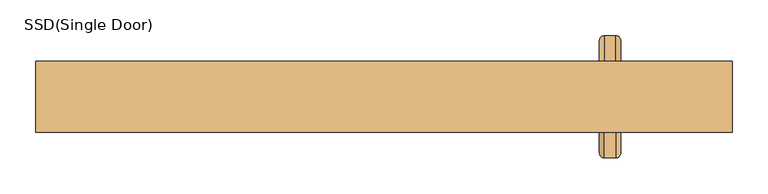
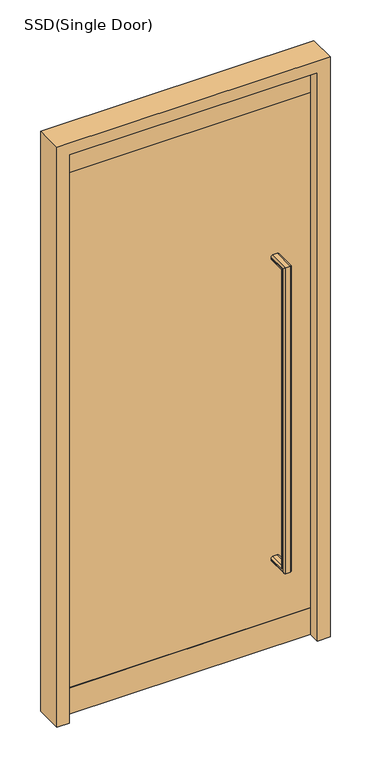
"""IFC4 building model written with IfcOpenShell, lengths in millimetres: door geometry, SSD(Single Door) : H_DR_AR B12_Door_Single_Glass_W1000xH2200_SSD-1."""

from ifc_helpers import new_model, si_unit, frame, origin, origin_with_axes, place, context, project, spatial, polyline, circle_curve, ellipse_curve, outline, extrude, source, transform, mapped, element, save
from ifc_brep_helpers import plane_surface, cylinder_surface, advanced_brep


def ssd_single_door_d0e6de12(model_context):
    return source(origin(), model_context, "Body", "SolidModel", [
        extrude(outline(polyline([(0.0, -490.0), (0.0, -445.0), (2155.0, -445.0), (2155.0, 445.0), (0.0, 445.0), (0.0, 490.0), (2200.0, 490.0), (2200.0, -490.0), (0.0, -490.0)])), frame((0.0, 5.0, 0.0), z_axis=(0.0, 1.0, 0.0), x_axis=(0.0, 0.0, 1.0)), (0.0, 0.0, 1.0), 100.0),
        advanced_brep(
        [(310.0, 49.0, 1485.0), (326.0, 49.0, 1485.0), (333.0, 49.0, 1478.0), (333.0, 49.0, 1475.0), (326.0, 49.0, 1468.0), (310.0, 49.0, 1468.0), (303.0, 49.0, 1475.0), (303.0, 49.0, 1478.0), (310.0, 49.0, 325.0), (303.0, 49.0, 332.0), (303.0, 49.0, 335.0), (310.0, 49.0, 342.0), (326.0, 49.0, 342.0), (333.0, 49.0, 335.0), (333.0, 49.0, 332.0), (326.0, 49.0, 325.0), (310.0, -31.0, 1485.0), (326.0, -31.0, 1485.0), (333.0, -24.0, 1478.0), (333.0, -24.0, 332.0), (333.0, -21.0, 335.0), (333.0, -21.0, 1475.0), (326.0, -14.0, 1468.0), (310.0, -14.0, 1468.0), (303.0, -21.0, 1475.0), (303.0, -21.0, 335.0), (303.0, -24.0, 332.0), (303.0, -24.0, 1478.0), (310.0, -31.0, 325.0), (326.0, -31.0, 325.0), (326.0, -14.0, 342.0), (310.0, -14.0, 342.0)],
        [
            (0, 1),
            (1, 2, circle_curve(frame((326.0, 49.0, 1478.0), z_axis=(0.0, 1.0, 0.0), x_axis=(0.0, 0.0, -1.0)), 7.0)),
            (2, 3),
            (3, 4, circle_curve(frame((326.0, 49.0, 1475.0), z_axis=(0.0, 1.0, 0.0), x_axis=(0.0, 0.0, -1.0)), 7.0)),
            (4, 5),
            (5, 6, circle_curve(frame((310.0, 49.0, 1475.0), z_axis=(0.0, 1.0, 0.0), x_axis=(0.0, 0.0, -1.0)), 7.0)),
            (6, 7),
            (7, 0, circle_curve(frame((310.0, 49.0, 1478.0), z_axis=(0.0, 1.0, 0.0), x_axis=(0.0, 0.0, -1.0)), 7.0)),
            (8, 9, circle_curve(frame((310.0, 49.0, 332.0), z_axis=(0.0, 1.0, 0.0), x_axis=(0.0, 0.0, 1.0)), 7.0)),
            (9, 10),
            (10, 11, circle_curve(frame((310.0, 49.0, 335.0), z_axis=(0.0, 1.0, 0.0), x_axis=(0.0, 0.0, 1.0)), 7.0)),
            (11, 12),
            (12, 13, circle_curve(frame((326.0, 49.0, 335.0), z_axis=(0.0, 1.0, 0.0), x_axis=(0.0, 0.0, 1.0)), 7.0)),
            (13, 14),
            (14, 15, circle_curve(frame((326.0, 49.0, 332.0), z_axis=(0.0, 1.0, 0.0), x_axis=(0.0, 0.0, 1.0)), 7.0)),
            (15, 8),
            (0, 16),
            (16, 17),
            (17, 1),
            (17, 18, ellipse_curve(frame((326.0, -24.0, 1478.0), z_axis=(0.0, 0.7071067811865475, 0.7071067811865475), x_axis=(0.0, 0.7071067811865476, -0.7071067811865474)), 9.8994949, 7.0)),
            (18, 2),
            (18, 19),
            (19, 14),
            (13, 20),
            (20, 21),
            (21, 3),
            (21, 22, ellipse_curve(frame((326.0, -21.0, 1475.0), z_axis=(0.0, 0.7071067811865475, 0.7071067811865475), x_axis=(0.0, 0.7071067811865476, -0.7071067811865474)), 9.8994949, 7.0)),
            (22, 4),
            (22, 23),
            (23, 5),
            (23, 24, ellipse_curve(frame((310.0, -21.0, 1475.0), z_axis=(0.0, 0.7071067811865475, 0.7071067811865475), x_axis=(0.0, 0.7071067811865476, -0.7071067811865474)), 9.8994949, 7.0)),
            (24, 6),
            (24, 25),
            (25, 10),
            (9, 26),
            (26, 27),
            (27, 7),
            (27, 16, ellipse_curve(frame((310.0, -24.0, 1478.0), z_axis=(0.0, 0.7071067811865475, 0.7071067811865475), x_axis=(0.0, 0.7071067811865476, -0.7071067811865474)), 9.8994949, 7.0)),
            (16, 28),
            (28, 29),
            (29, 17),
            (29, 19, ellipse_curve(frame((326.0, -24.0, 332.0), z_axis=(0.0, -0.7071067811865475, 0.7071067811865475), x_axis=(0.0, 0.7071067811865474, 0.7071067811865476)), 9.8994949, 7.0)),
            (20, 30, ellipse_curve(frame((326.0, -21.0, 335.0), z_axis=(0.0, -0.7071067811865475, 0.7071067811865475), x_axis=(0.0, 0.7071067811865474, 0.7071067811865476)), 9.8994949, 7.0)),
            (30, 22),
            (30, 31),
            (31, 23),
            (31, 25, ellipse_curve(frame((310.0, -21.0, 335.0), z_axis=(0.0, -0.7071067811865475, 0.7071067811865475), x_axis=(0.0, 0.7071067811865474, 0.7071067811865476)), 9.8994949, 7.0)),
            (26, 28, ellipse_curve(frame((310.0, -24.0, 332.0), z_axis=(0.0, -0.7071067811865475, 0.7071067811865475), x_axis=(0.0, 0.7071067811865474, 0.7071067811865476)), 9.8994949, 7.0)),
            (28, 8),
            (15, 29),
            (12, 30),
            (11, 31),
        ],
        [
            plane_surface(frame((0.0, 49.0, 1485.0), z_axis=(0.0, 1.0, 0.0), x_axis=(1.0, 0.0, 0.0))),
            plane_surface(frame((0.0, 49.0, 325.0), z_axis=(0.0, 1.0, 0.0), x_axis=(1.0, 0.0, 0.0))),
            plane_surface(frame((310.0, 49.0, 1485.0), z_axis=(0.0, 0.0, 1.0), x_axis=(0.0, -1.0, 0.0))),
            cylinder_surface(frame((326.0, 49.0, 1478.0), z_axis=(0.0, 1.0, 0.0), x_axis=(0.0, 0.0, -1.0)), 7.0),
            plane_surface(frame((333.0, 49.0, 1478.0), z_axis=(1.0, 0.0, 0.0), x_axis=(0.0, -1.0, 0.0))),
            cylinder_surface(frame((326.0, 49.0, 1475.0), z_axis=(0.0, 1.0, 0.0), x_axis=(0.0, 0.0, -1.0)), 7.0),
            plane_surface(frame((326.0, 49.0, 1468.0), z_axis=(0.0, 0.0, -1.0), x_axis=(0.0, -1.0, 0.0))),
            cylinder_surface(frame((310.0, 49.0, 1475.0), z_axis=(0.0, 1.0, 0.0), x_axis=(0.0, 0.0, -1.0)), 7.0),
            plane_surface(frame((303.0, 49.0, 1475.0), z_axis=(-1.0, 0.0, 0.0), x_axis=(0.0, -1.0, 0.0))),
            cylinder_surface(frame((310.0, 49.0, 1478.0), z_axis=(0.0, 1.0, 0.0), x_axis=(0.0, 0.0, -1.0)), 7.0),
            plane_surface(frame((310.0, -31.0, 1485.0), z_axis=(0.0, -1.0, 0.0), x_axis=(0.0, 0.0, -1.0))),
            cylinder_surface(frame((326.0, -24.0, 1485.0), z_axis=(0.0, 0.0, 1.0), x_axis=(0.0, 1.0, 0.0)), 7.0),
            cylinder_surface(frame((326.0, -21.0, 1485.0), z_axis=(0.0, 0.0, 1.0), x_axis=(0.0, 1.0, 0.0)), 7.0),
            plane_surface(frame((326.0, -14.0, 1468.0), z_axis=(0.0, 1.0, 0.0), x_axis=(0.0, 0.0, -1.0))),
            cylinder_surface(frame((310.0, -21.0, 1485.0), z_axis=(0.0, 0.0, 1.0), x_axis=(0.0, 1.0, 0.0)), 7.0),
            cylinder_surface(frame((310.0, -24.0, 1485.0), z_axis=(0.0, 0.0, 1.0), x_axis=(0.0, 1.0, 0.0)), 7.0),
            plane_surface(frame((310.0, -31.0, 325.0), z_axis=(0.0, 0.0, -1.0), x_axis=(0.0, 1.0, 0.0))),
            cylinder_surface(frame((326.0, -31.0, 332.0), z_axis=(0.0, -1.0, 0.0), x_axis=(0.0, 0.0, 1.0)), 7.0),
            cylinder_surface(frame((326.0, -31.0, 335.0), z_axis=(0.0, -1.0, 0.0), x_axis=(0.0, 0.0, 1.0)), 7.0),
            plane_surface(frame((326.0, -14.0, 342.0), z_axis=(0.0, 0.0, 1.0), x_axis=(0.0, 1.0, 0.0))),
            cylinder_surface(frame((310.0, -31.0, 335.0), z_axis=(0.0, -1.0, 0.0), x_axis=(0.0, 0.0, 1.0)), 7.0),
            cylinder_surface(frame((310.0, -31.0, 332.0), z_axis=(0.0, -1.0, 0.0), x_axis=(0.0, 0.0, 1.0)), 7.0),
        ],
        [
            (0, [[1, 2, 3, 4, 5, 6, 7, 8]]),
            (1, [[9, 10, 11, 12, 13, 14, 15, 16]]),
            (2, [[-1, 17, 18, 19]]),
            (3, [[-2, -19, 20, 21]]),
            (4, [[-3, -21, 22, 23, -14, 24, 25, 26]]),
            (5, [[-4, -26, 27, 28]]),
            (6, [[-5, -28, 29, 30]]),
            (7, [[-6, -30, 31, 32]]),
            (8, [[-7, -32, 33, 34, -10, 35, 36, 37]]),
            (9, [[-8, -37, 38, -17]]),
            (10, [[-18, 39, 40, 41]]),
            (11, [[-20, -41, 42, -22]]),
            (12, [[-27, -25, 43, 44]]),
            (13, [[-29, -44, 45, 46]]),
            (14, [[-31, -46, 47, -33]]),
            (15, [[-38, -36, 48, -39]]),
            (16, [[-40, 49, -16, 50]]),
            (17, [[-42, -50, -15, -23]]),
            (18, [[-43, -24, -13, 51]]),
            (19, [[-45, -51, -12, 52]]),
            (20, [[-47, -52, -11, -34]]),
            (21, [[-48, -35, -9, -49]]),
        ],
    ),
        advanced_brep(
        [(310.0, 61.0, 1485.0), (303.0, 61.0, 1478.0), (303.0, 61.0, 1475.0), (310.0, 61.0, 1468.0), (326.0, 61.0, 1468.0), (333.0, 61.0, 1475.0), (333.0, 61.0, 1478.0), (326.0, 61.0, 1485.0), (310.0, 61.0, 325.0), (326.0, 61.0, 325.0), (333.0, 61.0, 332.0), (333.0, 61.0, 335.0), (326.0, 61.0, 342.0), (310.0, 61.0, 342.0), (303.0, 61.0, 335.0), (303.0, 61.0, 332.0), (310.0, 141.0, 1485.0), (303.0, 134.0, 1478.0), (303.0, 134.0, 332.0), (303.0, 131.0, 335.0), (303.0, 131.0, 1475.0), (310.0, 124.0, 1468.0), (326.0, 124.0, 1468.0), (333.0, 131.0, 1475.0), (333.0, 131.0, 335.0), (333.0, 134.0, 332.0), (333.0, 134.0, 1478.0), (326.0, 141.0, 1485.0), (310.0, 141.0, 325.0), (310.0, 124.0, 342.0), (326.0, 124.0, 342.0), (326.0, 141.0, 325.0)],
        [
            (0, 1, circle_curve(frame((310.0, 61.0, 1478.0), z_axis=(0.0, -1.0, 0.0), x_axis=(0.0, 0.0, 1.0)), 7.0)),
            (1, 2),
            (2, 3, circle_curve(frame((310.0, 61.0, 1475.0), z_axis=(0.0, -1.0, 0.0), x_axis=(0.0, 0.0, 1.0)), 7.0)),
            (3, 4),
            (4, 5, circle_curve(frame((326.0, 61.0, 1475.0), z_axis=(0.0, -1.0, 0.0), x_axis=(0.0, 0.0, 1.0)), 7.0)),
            (5, 6),
            (6, 7, circle_curve(frame((326.0, 61.0, 1478.0), z_axis=(0.0, -1.0, 0.0), x_axis=(0.0, 0.0, 1.0)), 7.0)),
            (7, 0),
            (8, 9),
            (9, 10, circle_curve(frame((326.0, 61.0, 332.0), z_axis=(0.0, -1.0, 0.0), x_axis=(0.0, 0.0, -1.0)), 7.0)),
            (10, 11),
            (11, 12, circle_curve(frame((326.0, 61.0, 335.0), z_axis=(0.0, -1.0, 0.0), x_axis=(0.0, 0.0, -1.0)), 7.0)),
            (12, 13),
            (13, 14, circle_curve(frame((310.0, 61.0, 335.0), z_axis=(0.0, -1.0, 0.0), x_axis=(0.0, 0.0, -1.0)), 7.0)),
            (14, 15),
            (15, 8, circle_curve(frame((310.0, 61.0, 332.0), z_axis=(0.0, -1.0, 0.0), x_axis=(0.0, 0.0, -1.0)), 7.0)),
            (0, 16),
            (16, 17, ellipse_curve(frame((310.0, 134.0, 1478.0), z_axis=(0.0, -0.7071067811865475, 0.7071067811865475), x_axis=(0.0, -0.7071067811865476, -0.7071067811865474)), 9.8994949, 7.0)),
            (17, 1),
            (17, 18),
            (18, 15),
            (14, 19),
            (19, 20),
            (20, 2),
            (20, 21, ellipse_curve(frame((310.0, 131.0, 1475.0), z_axis=(0.0, -0.7071067811865475, 0.7071067811865475), x_axis=(0.0, -0.7071067811865476, -0.7071067811865474)), 9.8994949, 7.0)),
            (21, 3),
            (21, 22),
            (22, 4),
            (22, 23, ellipse_curve(frame((326.0, 131.0, 1475.0), z_axis=(0.0, -0.7071067811865475, 0.7071067811865475), x_axis=(0.0, -0.7071067811865476, -0.7071067811865474)), 9.8994949, 7.0)),
            (23, 5),
            (23, 24),
            (24, 11),
            (10, 25),
            (25, 26),
            (26, 6),
            (26, 27, ellipse_curve(frame((326.0, 134.0, 1478.0), z_axis=(0.0, -0.7071067811865475, 0.7071067811865475), x_axis=(0.0, -0.7071067811865476, -0.7071067811865474)), 9.8994949, 7.0)),
            (27, 7),
            (27, 16),
            (16, 28),
            (28, 18, ellipse_curve(frame((310.0, 134.0, 332.0), z_axis=(0.0, 0.7071067811865475, 0.7071067811865475), x_axis=(0.0, -0.7071067811865474, 0.7071067811865476)), 9.8994949, 7.0)),
            (19, 29, ellipse_curve(frame((310.0, 131.0, 335.0), z_axis=(0.0, 0.7071067811865475, 0.7071067811865475), x_axis=(0.0, -0.7071067811865474, 0.7071067811865476)), 9.8994949, 7.0)),
            (29, 21),
            (29, 30),
            (30, 22),
            (30, 24, ellipse_curve(frame((326.0, 131.0, 335.0), z_axis=(0.0, 0.7071067811865475, 0.7071067811865475), x_axis=(0.0, -0.7071067811865474, 0.7071067811865476)), 9.8994949, 7.0)),
            (25, 31, ellipse_curve(frame((326.0, 134.0, 332.0), z_axis=(0.0, 0.7071067811865475, 0.7071067811865475), x_axis=(0.0, -0.7071067811865474, 0.7071067811865476)), 9.8994949, 7.0)),
            (31, 27),
            (31, 28),
            (28, 8),
            (13, 29),
            (12, 30),
            (9, 31),
        ],
        [
            plane_surface(frame((0.0, 61.0, 1485.0), z_axis=(0.0, -1.0, 0.0), x_axis=(1.0, 0.0, 0.0))),
            plane_surface(frame((0.0, 61.0, 325.0), z_axis=(0.0, -1.0, 0.0), x_axis=(1.0, 0.0, 0.0))),
            cylinder_surface(frame((310.0, 61.0, 1478.0), z_axis=(0.0, -1.0, 0.0), x_axis=(0.0, 0.0, 1.0)), 7.0),
            plane_surface(frame((303.0, 61.0, 1478.0), z_axis=(-1.0, 0.0, 0.0), x_axis=(0.0, 1.0, 0.0))),
            cylinder_surface(frame((310.0, 61.0, 1475.0), z_axis=(0.0, -1.0, 0.0), x_axis=(0.0, 0.0, 1.0)), 7.0),
            plane_surface(frame((310.0, 61.0, 1468.0), z_axis=(0.0, 0.0, -1.0), x_axis=(0.0, 1.0, 0.0))),
            cylinder_surface(frame((326.0, 61.0, 1475.0), z_axis=(0.0, -1.0, 0.0), x_axis=(0.0, 0.0, 1.0)), 7.0),
            plane_surface(frame((333.0, 61.0, 1475.0), z_axis=(1.0, 0.0, 0.0), x_axis=(0.0, 1.0, 0.0))),
            cylinder_surface(frame((326.0, 61.0, 1478.0), z_axis=(0.0, -1.0, 0.0), x_axis=(0.0, 0.0, 1.0)), 7.0),
            plane_surface(frame((326.0, 61.0, 1485.0), z_axis=(0.0, 0.0, 1.0), x_axis=(0.0, 1.0, 0.0))),
            cylinder_surface(frame((310.0, 134.0, 1485.0), z_axis=(0.0, 0.0, 1.0), x_axis=(0.0, 1.0, 0.0)), 7.0),
            cylinder_surface(frame((310.0, 131.0, 1485.0), z_axis=(0.0, 0.0, 1.0), x_axis=(0.0, 1.0, 0.0)), 7.0),
            plane_surface(frame((310.0, 124.0, 1468.0), z_axis=(0.0, -1.0, 0.0), x_axis=(0.0, 0.0, -1.0))),
            cylinder_surface(frame((326.0, 131.0, 1485.0), z_axis=(0.0, 0.0, 1.0), x_axis=(0.0, 1.0, 0.0)), 7.0),
            cylinder_surface(frame((326.0, 134.0, 1485.0), z_axis=(0.0, 0.0, 1.0), x_axis=(0.0, 1.0, 0.0)), 7.0),
            plane_surface(frame((326.0, 141.0, 1485.0), z_axis=(0.0, 1.0, 0.0), x_axis=(0.0, 0.0, -1.0))),
            cylinder_surface(frame((310.0, 141.0, 332.0), z_axis=(0.0, 1.0, 0.0), x_axis=(0.0, 0.0, -1.0)), 7.0),
            cylinder_surface(frame((310.0, 141.0, 335.0), z_axis=(0.0, 1.0, 0.0), x_axis=(0.0, 0.0, -1.0)), 7.0),
            plane_surface(frame((310.0, 124.0, 342.0), z_axis=(0.0, 0.0, 1.0), x_axis=(0.0, -1.0, 0.0))),
            cylinder_surface(frame((326.0, 141.0, 335.0), z_axis=(0.0, 1.0, 0.0), x_axis=(0.0, 0.0, -1.0)), 7.0),
            cylinder_surface(frame((326.0, 141.0, 332.0), z_axis=(0.0, 1.0, 0.0), x_axis=(0.0, 0.0, -1.0)), 7.0),
            plane_surface(frame((326.0, 141.0, 325.0), z_axis=(0.0, 0.0, -1.0), x_axis=(0.0, -1.0, 0.0))),
        ],
        [
            (0, [[1, 2, 3, 4, 5, 6, 7, 8]]),
            (1, [[9, 10, 11, 12, 13, 14, 15, 16]]),
            (2, [[-1, 17, 18, 19]]),
            (3, [[-2, -19, 20, 21, -15, 22, 23, 24]]),
            (4, [[-3, -24, 25, 26]]),
            (5, [[-4, -26, 27, 28]]),
            (6, [[-5, -28, 29, 30]]),
            (7, [[-6, -30, 31, 32, -11, 33, 34, 35]]),
            (8, [[-7, -35, 36, 37]]),
            (9, [[-8, -37, 38, -17]]),
            (10, [[-18, 39, 40, -20]]),
            (11, [[-25, -23, 41, 42]]),
            (12, [[-27, -42, 43, 44]]),
            (13, [[-29, -44, 45, -31]]),
            (14, [[-36, -34, 46, 47]]),
            (15, [[-38, -47, 48, -39]]),
            (16, [[-40, 49, -16, -21]]),
            (17, [[-41, -22, -14, 50]]),
            (18, [[-43, -50, -13, 51]]),
            (19, [[-45, -51, -12, -32]]),
            (20, [[-46, -33, -10, 52]]),
            (21, [[-48, -52, -9, -49]]),
        ],
    ),
        extrude(outline(polyline([(445.0, 49.0), (-445.0, 49.0), (-445.0, 61.0), (445.0, 61.0), (445.0, 49.0)])), frame((0.0, 0.0, 100.0), z_axis=(0.0, 0.0, 1.0), x_axis=(1.0, 0.0, 0.0)), (0.0, 0.0, 1.0), 1955.0),
        extrude(outline(polyline([(445.0, 47.0), (-445.0, 47.0), (-445.0, 63.0), (445.0, 63.0), (445.0, 47.0)])), frame((0.0, 0.0, 2055.0), z_axis=(0.0, 0.0, 1.0), x_axis=(1.0, 0.0, 0.0)), (0.0, 0.0, 1.0), 100.0),
        extrude(outline(polyline([(445.0, 47.0), (-445.0, 47.0), (-445.0, 63.0), (445.0, 63.0), (445.0, 47.0)])), origin_with_axes(), (0.0, 0.0, 1.0), 100.0),
    ])


if __name__ == "__main__":
    model = new_model("IFC4")
    model_context = context("Model", 3, world=origin())
    ifc_project = project(units=[si_unit("LENGTHUNIT", "METRE", prefix="MILLI")], contexts=[model_context])
    site = spatial("IfcSite", under=ifc_project)
    building = spatial("IfcBuilding", under=site)
    placement = place(None, origin())
    ssd_single_door_shape = ssd_single_door_d0e6de12(model_context)
    element("IfcDoor", 1, ObjectType="SSD(Single Door) : H_DR_AR B12_Door_Single_Glass_W1000xH2200_SSD-1", at=placement, inside=building, context=model_context, shape_type="MappedRepresentation", body=[
        mapped(ssd_single_door_shape, transform((0.0, 0.0, 0.0), x_axis=(1.0, 0.0, 0.0), y_axis=(0.0, 1.0, 0.0), z_axis=(0.0, 0.0, 1.0))),
    ])
    save(model, "model.ifc")

# Revit data of these elements
# Type "SSD(Single Door) : H_DR_AR B12_Door_Single_Glass_W1000xH2200_SSD-1"
#   Type Mark = "452"
#   Type Comments = "SSD"
#   Analytic Construction = "<None>"
#   Thickness = 45 mm
#   Plan Door Swing2 = 890 mm
#   Plan Door Swing = 1780 mm
#   Glass Thk = 12 mm
#   Frame THK = 100 mm
#   Frame Projection Ext. = 25 mm
#   Frame Projection Int. = 25 mm
#   Frame Width = 75 mm
#   Height = 2200 mm
#   Width = 980 mm
#   Center Door [instance default] = 100 mm
#   Define Thermal Properties by = 1
#   Function = (empty or 0)
#   Wall Closure = (empty or 0)
# Element 1 (IfcDoor, "SSD(Single Door) : H_DR_AR B12_Door_Single_Glass_W1000xH2200_SSD-1")
#   Center Door = 55 mm
#   Materials on its faces: "Stainless Steel", "Glass"
# Materials
#   "Stainless Steel": class "Metal", colour RGB 189 187 185, transparency 0, Description = "Stainless Steel 18/8", Cost = 0
#   "Glass": class "Glass", colour RGB 218 227 224, transparency 0.85, Description = "Soda Lime Glass", Cost = 0
